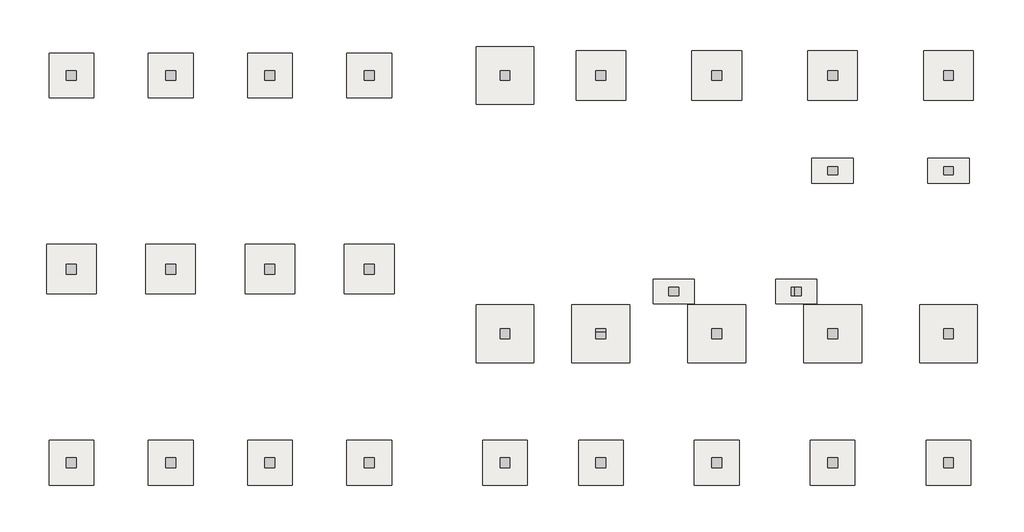
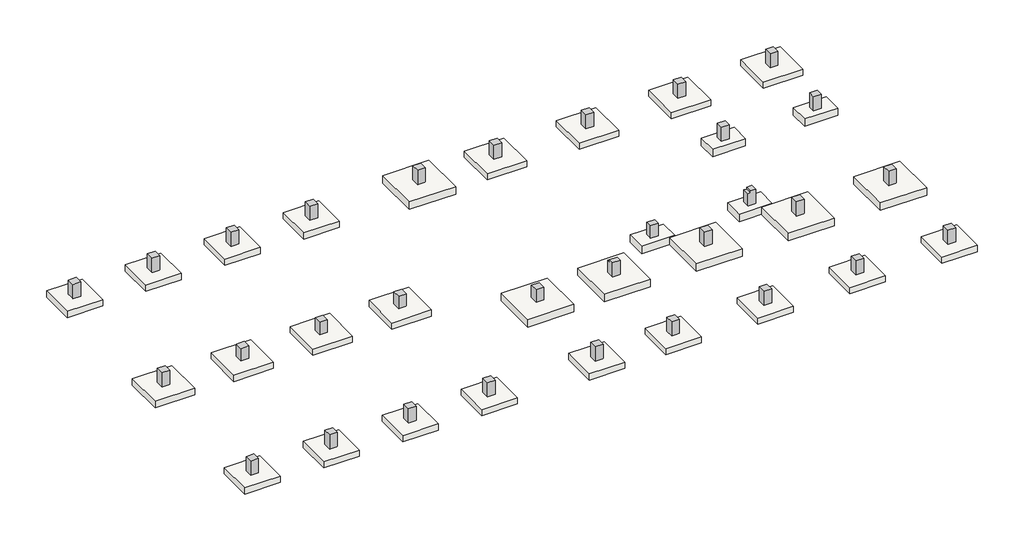
# Not in any storey: 31 columns, 31 slabs.
"""IFC4 building model written with IfcOpenShell, lengths in millimetres."""

import ifcopenshell
import ifcopenshell.guid

model = None  # the IFC model being written
_history = None  # IfcOwnerHistory: only IFC2X3 demands one
_inside = {}  # id of a spatial element -> (the spatial element, [elements in it])
_under = {}  # id of a project, library or spatial element -> (it, [spatial elements below it])
_declared = {}  # id of a project -> (the project, [libraries it declares])
_typed = {}  # id of a type object -> (the type object, [elements of that type])
_made_of = {}  # id of a material, layer set ... -> (it, [elements and type objects made of it])


def new_model(schema):
    """Start an empty IFC model of exactly this schema.

    Asked for "IFC4X3", IfcOpenShell would pick the latest addendum, in which some entities
    have other attributes; the version numbers below select the first issue.
    IFC2X3 requires an IfcOwnerHistory on every rooted entity: one is made here for all.
    """
    global model, _history
    if schema == "IFC4X3":
        model = ifcopenshell.file(schema_version=(4, 3, 0, 0))
    else:
        model = ifcopenshell.file(schema=schema)
    _inside.clear()
    _under.clear()
    _declared.clear()
    _typed.clear()
    _made_of.clear()
    _history = None
    if model.schema == "IFC2X3":
        org = make("IfcOrganization", Name="unknown")
        user = make(
            "IfcPersonAndOrganization",
            ThePerson=make("IfcPerson", FamilyName="unknown"),
            TheOrganization=org,
        )
        app = make(
            "IfcApplication",
            ApplicationDeveloper=org,
            Version="unknown",
            ApplicationFullName="unknown",
            ApplicationIdentifier="unknown",
        )
        _history = make(
            "IfcOwnerHistory",
            OwningUser=user,
            OwningApplication=app,
            ChangeAction="ADDED",
            CreationDate=0,
        )
    return model


def make(cls, **values):
    """One entity of the class cls with the attributes given. An attribute that is None is left unset."""
    return model.create_entity(
        cls, **{name: value for name, value in values.items() if value is not None}
    )


def rooted(cls, **values):
    """An entity with a GlobalId (a new one), such as an element, a storey or a relation."""
    return make(cls, GlobalId=ifcopenshell.guid.new(), OwnerHistory=_history, **values)


def si_unit(unit_type, name, prefix=None):
    """IfcSIUnit, for example si_unit("LENGTHUNIT", "METRE", prefix="MILLI")."""
    return make("IfcSIUnit", UnitType=unit_type, Prefix=prefix, Name=name)


def assignment(units):
    """IfcUnitAssignment: the units of a project."""
    return None if units is None else make("IfcUnitAssignment", Units=units)


def point(xyz):
    """IfcCartesianPoint."""
    return None if xyz is None else make("IfcCartesianPoint", Coordinates=xyz)


def direction(xyz):
    """IfcDirection."""
    return None if xyz is None else make("IfcDirection", DirectionRatios=xyz)


def frame(location, z_axis=None, x_axis=None):
    """IfcAxis2Placement3D, a coordinate frame: its origin and axes. An axis left out is left unset."""
    return make(
        "IfcAxis2Placement3D",
        Location=point(location),
        Axis=direction(z_axis),
        RefDirection=direction(x_axis),
    )


def origin():
    """The frame at (0, 0, 0) with its axes left unset."""
    return frame((0.0, 0.0, 0.0))


def place(relative_to, where):
    """IfcLocalPlacement: puts the frame where relative to a parent placement (None: the world)."""
    return make(
        "IfcLocalPlacement", PlacementRelTo=relative_to, RelativePlacement=where
    )


def context(
    kind, dimensions, precision=None, world=None, true_north=None, identifier=None
):
    """IfcGeometricRepresentationContext, for example the 3D "Model" context."""
    return make(
        "IfcGeometricRepresentationContext",
        ContextIdentifier=identifier,
        ContextType=kind,
        CoordinateSpaceDimension=dimensions,
        Precision=precision,
        WorldCoordinateSystem=world,
        TrueNorth=true_north,
    )


def project(units=None, contexts=None):
    """IfcProject with its units and contexts."""
    return rooted(
        "IfcProject",
        Name="project",
        RepresentationContexts=contexts,
        UnitsInContext=assignment(units),
    )


def spatial(cls, under=None, at=None, **own):
    """A site, building, storey or space (cls), placed at a placement, below another one or the project."""
    s = rooted(cls, ObjectPlacement=at, **own)
    if under is not None:
        _under.setdefault(under.id(), (under, []))[1].append(s)
    return s


def polyline(points):
    """IfcPolyline through the points."""
    return make("IfcPolyline", Points=[point(p) for p in points])


def outline(outer, holes=None, kind="AREA"):
    """IfcArbitraryClosedProfileDef: a profile drawn as a closed curve; with holes, ...WithVoids."""
    if holes is None:
        return make("IfcArbitraryClosedProfileDef", ProfileType=kind, OuterCurve=outer)
    return make(
        "IfcArbitraryProfileDefWithVoids",
        ProfileType=kind,
        OuterCurve=outer,
        InnerCurves=holes,
    )


def extrude(swept, where, along, depth):
    """IfcExtrudedAreaSolid: the profile swept, set in the frame where, extruded along a direction by depth."""
    return make(
        "IfcExtrudedAreaSolid",
        SweptArea=swept,
        Position=where,
        ExtrudedDirection=direction(along),
        Depth=depth,
    )


def faces_of(points, faces, orient=None, outer=None):
    """IfcFace entities. A face is a list of loops; a loop is a list of indices into points, from 0.

    orient and outer hold one flag for each loop. By default every Orientation is true, the
    first loop of a face is its IfcFaceOuterBound and the others are IfcFaceBound.
    """
    made = []
    for i, loops in enumerate(faces):
        bounds = []
        for j, loop in enumerate(loops):
            is_outer = j == 0 if outer is None else outer[i][j]
            bounds.append(
                make(
                    "IfcFaceOuterBound" if is_outer else "IfcFaceBound",
                    Bound=make("IfcPolyLoop", Polygon=[points[k] for k in loop]),
                    Orientation=True if orient is None else orient[i][j],
                )
            )
        made.append(make("IfcFace", Bounds=bounds))
    return made


def faceted_brep(points, faces, orient=None, outer=None, voids=None):
    """IfcFacetedBrep: a solid bounded by flat faces; with voids (closed shells), ...WithVoids."""
    shared = [point(p) for p in points]
    hull = make("IfcClosedShell", CfsFaces=faces_of(shared, faces, orient, outer))
    if voids is None:
        return make("IfcFacetedBrep", Outer=hull)
    return make(
        "IfcFacetedBrepWithVoids",
        Outer=hull,
        Voids=[
            make(cls, CfsFaces=faces_of(shared, fs, o, b)) for cls, fs, o, b in voids
        ],
    )


def shape(context_of_items, identifier, shape_type, items):
    """IfcShapeRepresentation: the items that make up one representation, for example the "Body"."""
    return make(
        "IfcShapeRepresentation",
        ContextOfItems=context_of_items,
        RepresentationIdentifier=identifier,
        RepresentationType=shape_type,
        Items=items,
    )


def made_of(thing, what):
    """Note that an element or type object is made of a material, layer set ...; save() writes the relation."""
    if what is not None:
        _made_of.setdefault(what.id(), (what, []))[1].append(thing)
    return thing


def element(
    cls,
    number,
    at=None,
    inside=None,
    cuts=None,
    type_object=None,
    material=None,
    context=None,
    identifier="Body",
    shape_type=None,
    held_by="IfcProductDefinitionShape",
    body=None,
    shapes=None,
    **own,
):
    """One element of the class cls, such as IfcWall. Its Tag is "e" and its number.

    at: its placement. inside: the storey or other place that contains it. cuts: it is an
    opening in that element (IfcRelVoidsElement). A single representation is given by context,
    identifier, shape_type and body (its items); several are given by shapes. held_by: the class
    of the entity that holds the representations. save() writes the other relations.
    """
    e = rooted(cls, Tag="e%d" % number, ObjectPlacement=at, **own)
    if body is not None:
        shapes = [shape(context, identifier, shape_type, body)]
    if shapes is not None:
        e.Representation = make(held_by, Representations=shapes)
    if inside is not None:
        _inside.setdefault(inside.id(), (inside, []))[1].append(e)
    if cuts is not None:
        rooted(
            "IfcRelVoidsElement", RelatingBuildingElement=cuts, RelatedOpeningElement=e
        )
    if type_object is not None:
        _typed.setdefault(type_object.id(), (type_object, []))[1].append(e)
    return made_of(e, material)


def aggregate(whole, parts):
    """IfcRelAggregates: a whole, such as a stair, and the parts it consists of."""
    return rooted("IfcRelAggregates", RelatingObject=whole, RelatedObjects=parts)


def save(model, path):
    """Write the relations noted so far, then the file.

    IfcRelAggregates (storeys below a building ...), IfcRelContainedInSpatialStructure (elements
    in a storey), IfcRelDefinesByType, IfcRelAssociatesMaterial and IfcRelDeclares: one each for
    every whole, place, type object, material and project.
    """
    for whole, parts in _under.values():
        aggregate(whole, parts)
    for where, things in _inside.values():
        rooted(
            "IfcRelContainedInSpatialStructure",
            RelatedElements=things,
            RelatingStructure=where,
        )
    for kind, things in _typed.values():
        rooted("IfcRelDefinesByType", RelatedObjects=things, RelatingType=kind)
    for what, things in _made_of.values():
        rooted("IfcRelAssociatesMaterial", RelatedObjects=things, RelatingMaterial=what)
    for by, libraries in _declared.values():
        rooted("IfcRelDeclares", RelatingContext=by, RelatedDefinitions=libraries)
    model.write(path)


model = new_model("IFC4")

# Units and contexts
model_context = context("Model", 3, world=origin())
ifc_project = project(units=[si_unit("LENGTHUNIT", "METRE", prefix="MILLI")], contexts=[model_context])

# Site, building
site = spatial("IfcSite", under=ifc_project)
building = spatial("IfcBuilding", under=site)

# Columns
placement = place(None, origin())
element("IfcColumn", 1, ObjectType="RC_Column_Rectangular : H_SC_AR_S15_UG PED_W600xL600_Bit", at=placement, inside=building, context=model_context, shape_type="Brep", body=[
    faceted_brep([(300.0, 12499.5208589, -1150.0381366), (300.0, 11899.5208589, -1150.0381366), (-300.0, 11899.5208589, -1150.0381366), (-300.0, 12499.5208589, -1150.0381366), (300.0, 12499.5208589, -0.0381366), (300.0, 11899.5208589, -0.0381366), (300.0, 11899.5208589, -150.0381366), (300.0, 11899.5208589, -650.0381366), (300.0, 12499.5208589, -650.0381366), (300.0, 12499.5208589, -150.0381366), (-300.0, 11899.5208589, -0.0381366), (-300.0, 11899.5208589, -150.0381366), (-300.0, 11899.5208589, -650.0381366), (-300.0, 12499.5208589, -0.0381366), (-300.0, 12499.5208589, -150.0381366), (-300.0, 12499.5208589, -650.0381366)], [[[0, 1, 2, 3]], [[4, 5, 6, 7, 1, 0, 8, 9]], [[5, 10, 11, 12, 2, 1, 7, 6]], [[10, 13, 14, 15, 3, 2, 12, 11]], [[13, 4, 9, 8, 0, 3, 15, 14]], [[4, 13, 10, 5]]]),
])
element("IfcColumn", 2, ObjectType="RC_Column_Rectangular : H_SC_AR_S15_UG PED_W600xL600_Bit", at=placement, inside=building, context=model_context, shape_type="SweptSolid", body=[
    extrude(outline(polyline([(6300.0, 12499.5208589), (6300.0, 11899.5208589), (5700.0, 11899.5208589), (5700.0, 12499.5208589), (6300.0, 12499.5208589)])), frame((0.0, 0.0, -1150.0381366), z_axis=(0.0, 0.0, 1.0), x_axis=(1.0, 0.0, 0.0)), (0.0, 0.0, 1.0), 1000.0),
])
element("IfcColumn", 3, ObjectType="RC_Column_Rectangular : H_SC_AR_S15_UG PED_W600xL600_Bit", at=placement, inside=building, context=model_context, shape_type="SweptSolid", body=[
    extrude(outline(polyline([(12300.0, 12499.5208589), (12300.0, 11899.5208589), (11700.0, 11899.5208589), (11700.0, 12499.5208589), (12300.0, 12499.5208589)])), frame((0.0, 0.0, -1150.0381366), z_axis=(0.0, 0.0, 1.0), x_axis=(1.0, 0.0, 0.0)), (0.0, 0.0, 1.0), 1000.0),
])
element("IfcColumn", 4, ObjectType="RC_Column_Rectangular : H_SC_AR_S15_UG PED_W600xL600_Bit", at=placement, inside=building, context=model_context, shape_type="Brep", body=[
    faceted_brep([(18300.0, 12499.5208589, -1150.0381366), (18300.0, 11899.5208589, -1150.0381366), (17700.0, 11899.5208589, -1150.0381366), (17700.0, 12499.5208589, -1150.0381366), (18300.0, 12499.5208589, -150.0381366), (18300.0, 11899.5208589, -150.0381366), (18200.0, 11899.5208589, -150.0381366), (17700.0, 11899.5208589, -150.0381366), (17700.0, 12499.5208589, -150.0381366)], [[[0, 1, 2, 3]], [[1, 0, 4, 5]], [[2, 1, 5, 6, 7]], [[3, 2, 7, 8]], [[0, 3, 8, 4]], [[5, 4, 8, 7, 6]]]),
])
element("IfcColumn", 5, ObjectType="RC_Column_Rectangular : H_SC_AR_S15_UG PED_W600xL600_Bit", at=placement, inside=building, context=model_context, shape_type="Brep", body=[
    faceted_brep([(300.0, 24199.5208589, -1150.0381366), (300.0, 23599.5208589, -1150.0381366), (-300.0, 23599.5208589, -1150.0381366), (-300.0, 24199.5208589, -1150.0381366), (300.0, 24199.5208589, -0.0381366), (300.0, 23599.5208589, -0.0381366), (300.0, 23599.5208589, -150.0381366), (300.0, 23599.5208589, -650.0381366), (300.0, 24199.5208589, -650.0381366), (300.0, 24199.5208589, -150.0381366), (-300.0, 23599.5208589, -0.0381366), (-300.0, 23599.5208589, -150.0381366), (-300.0, 23599.5208589, -650.0381366), (-300.0, 24199.5208589, -0.0381366)], [[[0, 1, 2, 3]], [[4, 5, 6, 7, 1, 0, 8, 9]], [[5, 10, 11, 12, 2, 1, 7, 6]], [[10, 13, 3, 2, 12, 11]], [[13, 4, 9, 8, 0, 3]], [[4, 13, 10, 5]]]),
])
element("IfcColumn", 6, ObjectType="RC_Column_Rectangular : H_SC_AR_S15_UG PED_W600xL600_Bit", at=placement, inside=building, context=model_context, shape_type="Brep", body=[
    faceted_brep([(6300.0, 24199.5208589, -1150.0381366), (6300.0, 23599.5208589, -1150.0381366), (5700.0, 23599.5208589, -1150.0381366), (5700.0, 24199.5208589, -1150.0381366), (6300.0, 24199.5208589, -0.0381366), (6300.0, 23599.5208589, -0.0381366), (6300.0, 23599.5208589, -150.0381366), (6300.0, 23599.5208589, -650.0381366), (6300.0, 24199.5208589, -650.0381366), (6300.0, 24199.5208589, -150.0381366), (5700.0, 23599.5208589, -0.0381366), (5700.0, 23599.5208589, -150.0381366), (5700.0, 23599.5208589, -650.0381366), (5700.0, 24199.5208589, -0.0381366), (5700.0, 24199.5208589, -150.0381366), (5700.0, 24199.5208589, -650.0381366)], [[[0, 1, 2, 3]], [[4, 5, 6, 7, 1, 0, 8, 9]], [[5, 10, 11, 12, 2, 1, 7, 6]], [[10, 13, 14, 15, 3, 2, 12, 11]], [[13, 4, 9, 8, 0, 3, 15, 14]], [[4, 13, 10, 5]]]),
])
element("IfcColumn", 7, ObjectType="RC_Column_Rectangular : H_SC_AR_S15_UG PED_W600xL600_Bit", at=placement, inside=building, context=model_context, shape_type="Brep", body=[
    faceted_brep([(12300.0, 24199.5208589, -1150.0381366), (12300.0, 23599.5208589, -1150.0381366), (11700.0, 23599.5208589, -1150.0381366), (11700.0, 24199.5208589, -1150.0381366), (12300.0, 24199.5208589, -0.0381366), (12300.0, 23599.5208589, -0.0381366), (12300.0, 23599.5208589, -150.0381366), (12300.0, 23599.5208589, -650.0381366), (12300.0, 24199.5208589, -650.0381366), (12300.0, 24199.5208589, -150.0381366), (11700.0, 23599.5208589, -0.0381366), (11700.0, 23599.5208589, -150.0381366), (11700.0, 23599.5208589, -650.0381366), (11700.0, 24199.5208589, -0.0381366), (11700.0, 24199.5208589, -150.0381366), (11700.0, 24199.5208589, -650.0381366)], [[[0, 1, 2, 3]], [[4, 5, 6, 7, 1, 0, 8, 9]], [[5, 10, 11, 12, 2, 1, 7, 6]], [[10, 13, 14, 15, 3, 2, 12, 11]], [[13, 4, 9, 8, 0, 3, 15, 14]], [[4, 13, 10, 5]]]),
])
element("IfcColumn", 8, ObjectType="RC_Column_Rectangular : H_SC_AR_S15_UG PED_W600xL600_Bit", at=placement, inside=building, context=model_context, shape_type="Brep", body=[
    faceted_brep([(18300.0, 24199.5208589, -1150.0381366), (18300.0, 23599.5208589, -1150.0381366), (17700.0, 23599.5208589, -1150.0381366), (17700.0, 24199.5208589, -1150.0381366), (18300.0, 24199.5208589, -0.0381366), (18300.0, 23599.5208589, -0.0381366), (18300.0, 23599.5208589, -150.0381366), (18300.0, 23599.5208589, -650.0381366), (18300.0, 24199.5208589, -650.0381366), (18300.0, 24199.5208589, -150.0381366), (17700.0, 23599.5208589, -0.0381366), (17700.0, 23599.5208589, -150.0381366), (17700.0, 23599.5208589, -650.0381366), (17700.0, 24199.5208589, -0.0381366), (17700.0, 24199.5208589, -150.0381366), (17700.0, 24199.5208589, -650.0381366)], [[[0, 1, 2, 3]], [[4, 5, 6, 7, 1, 0, 8, 9]], [[5, 10, 11, 12, 2, 1, 7, 6]], [[10, 13, 14, 15, 3, 2, 12, 11]], [[13, 4, 9, 8, 0, 3, 15, 14]], [[4, 13, 10, 5]]]),
])
element("IfcColumn", 9, ObjectType="RC_Column_Rectangular : H_SC_AR_S15_UG PED_W600xL600_Bit", at=placement, inside=building, context=model_context, shape_type="Brep", body=[
    faceted_brep([(26500.0, 24199.5208589, -1150.0381366), (26500.0, 23599.5208589, -1150.0381366), (25900.0, 23599.5208589, -1150.0381366), (25900.0, 24199.5208589, -1150.0381366), (26500.0, 24199.5208589, -0.0381366), (26500.0, 23599.5208589, -0.0381366), (26500.0, 23599.5208589, -150.0381366), (26500.0, 23599.5208589, -650.0381366), (26500.0, 24199.5208589, -650.0381366), (26500.0, 24199.5208589, -150.0381366), (25900.0, 23599.5208589, -0.0381366), (25900.0, 23599.5208589, -150.0381366), (25900.0, 23599.5208589, -650.0381366), (25900.0, 24199.5208589, -0.0381366), (25900.0, 24199.5208589, -150.0381366), (25900.0, 24199.5208589, -650.0381366)], [[[0, 1, 2, 3]], [[4, 5, 6, 7, 1, 0, 8, 9]], [[5, 10, 11, 12, 2, 1, 7, 6]], [[10, 13, 14, 15, 3, 2, 12, 11]], [[13, 4, 9, 8, 0, 3, 15, 14]], [[4, 13, 10, 5]]]),
])
element("IfcColumn", 10, ObjectType="RC_Column_Rectangular : H_SC_AR_S15_UG PED_W600xL600_Bit", at=placement, inside=building, context=model_context, shape_type="Brep", body=[
    faceted_brep([(32300.0, 24199.5208589, -1150.0381366), (32300.0, 23599.5208589, -1150.0381366), (31700.0, 23599.5208589, -1150.0381366), (31700.0, 24199.5208589, -1150.0381366), (32300.0, 24199.5208589, -0.0381366), (32300.0, 23599.5208589, -0.0381366), (32300.0, 23599.5208589, -150.0381366), (32300.0, 23599.5208589, -650.0381366), (32300.0, 24199.5208589, -650.0381366), (32300.0, 24199.5208589, -150.0381366), (31700.0, 23599.5208589, -0.0381366), (31700.0, 23599.5208589, -150.0381366), (31700.0, 23599.5208589, -650.0381366), (31700.0, 24199.5208589, -0.0381366), (31700.0, 24199.5208589, -150.0381366), (31700.0, 24199.5208589, -650.0381366)], [[[0, 1, 2, 3]], [[4, 5, 6, 7, 1, 0, 8, 9]], [[5, 10, 11, 12, 2, 1, 7, 6]], [[10, 13, 14, 15, 3, 2, 12, 11]], [[13, 4, 9, 8, 0, 3, 15, 14]], [[4, 13, 10, 5]]]),
])
element("IfcColumn", 11, ObjectType="RC_Column_Rectangular : H_SC_AR_S15_UG PED_W600xL600_Bit", at=placement, inside=building, context=model_context, shape_type="Brep", body=[
    faceted_brep([(39300.0, 24199.5208589, -1150.0381366), (39300.0, 23599.5208589, -1150.0381366), (38700.0, 23599.5208589, -1150.0381366), (38700.0, 24199.5208589, -1150.0381366), (39300.0, 24199.5208589, -0.0381366), (39300.0, 23599.5208589, -0.0381366), (39300.0, 23599.5208589, -150.0381366), (39300.0, 23599.5208589, -650.0381366), (39300.0, 24199.5208589, -650.0381366), (39300.0, 24199.5208589, -150.0381366), (38700.0, 23599.5208589, -0.0381366), (38700.0, 23599.5208589, -150.0381366), (38700.0, 23599.5208589, -650.0381366), (38700.0, 24199.5208589, -0.0381366), (38700.0, 24199.5208589, -150.0381366), (38700.0, 24199.5208589, -650.0381366)], [[[0, 1, 2, 3]], [[4, 5, 6, 7, 1, 0, 8, 9]], [[5, 10, 11, 12, 2, 1, 7, 6]], [[10, 13, 14, 15, 3, 2, 12, 11]], [[13, 4, 9, 8, 0, 3, 15, 14]], [[4, 13, 10, 5]]]),
])
element("IfcColumn", 12, ObjectType="RC_Column_Rectangular : H_SC_AR_S15_UG PED_W600xL600_Bit", at=placement, inside=building, context=model_context, shape_type="Brep", body=[
    faceted_brep([(46300.0, 24199.5208589, -1150.0381366), (46300.0, 23599.5208589, -1150.0381366), (45700.0, 23599.5208589, -1150.0381366), (45700.0, 24199.5208589, -1150.0381366), (46300.0, 24199.5208589, -0.0381366), (46300.0, 23599.5208589, -0.0381366), (46300.0, 23599.5208589, -150.0381366), (46300.0, 23599.5208589, -650.0381366), (46300.0, 24199.5208589, -650.0381366), (46300.0, 24199.5208589, -150.0381366), (45700.0, 23599.5208589, -0.0381366), (45700.0, 23599.5208589, -150.0381366), (45700.0, 23599.5208589, -650.0381366), (45700.0, 24199.5208589, -0.0381366), (45700.0, 24199.5208589, -150.0381366), (45700.0, 24199.5208589, -650.0381366)], [[[0, 1, 2, 3]], [[4, 5, 6, 7, 1, 0, 8, 9]], [[5, 10, 11, 12, 2, 1, 7, 6]], [[10, 13, 14, 15, 3, 2, 12, 11]], [[13, 4, 9, 8, 0, 3, 15, 14]], [[4, 13, 10, 5]]]),
])
element("IfcColumn", 13, ObjectType="RC_Column_Rectangular : H_SC_AR_S15_UG PED_W600xL600_Bit", at=placement, inside=building, context=model_context, shape_type="Brep", body=[
    faceted_brep([(53300.0, 24199.5208589, -1150.0381366), (53300.0, 23599.5208589, -1150.0381366), (52700.0, 23599.5208589, -1150.0381366), (52700.0, 24199.5208589, -1150.0381366), (53300.0, 24199.5208589, -0.0381366), (53300.0, 23599.5208589, -0.0381366), (53300.0, 23599.5208589, -150.0381366), (53300.0, 23599.5208589, -650.0381366), (52700.0, 23599.5208589, -0.0381366), (52700.0, 23599.5208589, -150.0381366), (52700.0, 23599.5208589, -650.0381366), (52700.0, 24199.5208589, -0.0381366), (52700.0, 24199.5208589, -150.0381366), (52700.0, 24199.5208589, -650.0381366)], [[[0, 1, 2, 3]], [[4, 5, 6, 7, 1, 0]], [[5, 8, 9, 10, 2, 1, 7, 6]], [[8, 11, 12, 13, 3, 2, 10, 9]], [[11, 4, 0, 3, 13, 12]], [[4, 11, 8, 5]]]),
])
element("IfcColumn", 14, ObjectType="RC_Column_Rectangular : H_SC_AR_S15_UG PED_W600xL600_Bit", at=placement, inside=building, context=model_context, shape_type="Brep", body=[
    faceted_brep([(26500.0, 8599.5208589, -1150.0381366), (26500.0, 7999.5208589, -1150.0381366), (25900.0, 7999.5208589, -1150.0381366), (25900.0, 8599.5208589, -1150.0381366), (26500.0, 8599.5208589, -150.0381366), (26500.0, 8399.5208589, -150.0381366), (26500.0, 7999.5208589, -150.0381366), (25900.0, 7999.5208589, -150.0381366), (25900.0, 8599.5208589, -150.0381366)], [[[0, 1, 2, 3]], [[1, 0, 4, 5, 6]], [[2, 1, 6, 7]], [[3, 2, 7, 8]], [[0, 3, 8, 4]], [[4, 8, 7, 6, 5]]]),
])
element("IfcColumn", 15, ObjectType="RC_Column_Rectangular : H_SC_AR_S15_UG PED_W600xL600_Bit", at=placement, inside=building, context=model_context, shape_type="Brep", body=[
    faceted_brep([(32300.0, 8599.5208589, -1150.0381366), (32300.0, 7999.5208589, -1150.0381366), (31700.0, 7999.5208589, -1150.0381366), (31700.0, 8599.5208589, -1150.0381366), (32300.0, 8599.5208589, -150.0381366), (32300.0, 8399.5208589, -150.0381366), (32300.0, 8399.5208589, -0.0381366), (32300.0, 7999.5208589, -0.0381366), (31700.0, 7999.5208589, -0.0381366), (31700.0, 8399.5208589, -0.0381366), (31700.0, 8399.5208589, -150.0381366), (31700.0, 8599.5208589, -150.0381366), (31800.0, 8399.5208589, -0.0381366), (31800.0, 8399.5208589, -150.0381366)], [[[0, 1, 2, 3]], [[1, 0, 4, 5, 6, 7]], [[2, 1, 7, 8]], [[3, 2, 8, 9, 10, 11]], [[0, 3, 11, 4]], [[8, 7, 6, 12, 9]], [[10, 13, 5, 4, 11]], [[5, 13, 12, 6]], [[13, 10, 9, 12]]]),
])
element("IfcColumn", 16, ObjectType="RC_Column_Rectangular : H_SC_AR_S15_UG PED_W600xL600_Bit", at=placement, inside=building, context=model_context, shape_type="SweptSolid", body=[
    extrude(outline(polyline([(39300.0, 8599.5208589), (39300.0, 7999.5208589), (38700.0, 7999.5208589), (38700.0, 8599.5208589), (39300.0, 8599.5208589)])), frame((0.0, 0.0, -1150.0381366), z_axis=(0.0, 0.0, 1.0), x_axis=(1.0, 0.0, 0.0)), (0.0, 0.0, 1.0), 1150.0),
])
element("IfcColumn", 17, ObjectType="RC_Column_Rectangular : H_SC_AR_S15_UG PED_W600xL600_Bit", at=placement, inside=building, context=model_context, shape_type="SweptSolid", body=[
    extrude(outline(polyline([(46300.0, 8599.5208589), (46300.0, 7999.5208589), (45700.0, 7999.5208589), (45700.0, 8599.5208589), (46300.0, 8599.5208589)])), frame((0.0, 0.0, -1150.0381366), z_axis=(0.0, 0.0, 1.0), x_axis=(1.0, 0.0, 0.0)), (0.0, 0.0, 1.0), 1150.0),
])
element("IfcColumn", 18, ObjectType="RC_Column_Rectangular : H_SC_AR_S15_UG PED_W600xL600_Bit", at=placement, inside=building, context=model_context, shape_type="Brep", body=[
    faceted_brep([(53300.0, 8599.5208589, -1150.0381366), (53300.0, 7999.5208589, -1150.0381366), (52700.0, 7999.5208589, -1150.0381366), (52700.0, 8599.5208589, -1150.0381366), (53300.0, 8599.5208589, -0.0381366), (53300.0, 7999.5208589, -0.0381366), (53300.0, 7999.5208589, -150.0381366), (53300.0, 7999.5208589, -650.0381366), (53300.0, 8599.5208589, -650.0381366), (53300.0, 8599.5208589, -150.0381366), (52700.0, 7999.5208589, -0.0381366), (52700.0, 7999.5208589, -150.0381366), (52700.0, 7999.5208589, -650.0381366), (52700.0, 8599.5208589, -0.0381366), (52700.0, 8599.5208589, -150.0381366), (52700.0, 8599.5208589, -650.0381366)], [[[0, 1, 2, 3]], [[4, 5, 6, 7, 1, 0, 8, 9]], [[5, 10, 11, 12, 2, 1, 7, 6]], [[10, 13, 14, 15, 3, 2, 12, 11]], [[13, 4, 9, 8, 0, 3, 15, 14]], [[4, 13, 10, 5]]]),
])
element("IfcColumn", 19, ObjectType="RC_Column_Rectangular : H_SC_AR_S15_UG PED_W600xL600_Bit", at=placement, inside=building, context=model_context, shape_type="Brep", body=[
    faceted_brep([(300.0, 799.5208589, -1150.0381366), (300.0, 199.5208589, -1150.0381366), (-300.0, 199.5208589, -1150.0381366), (-300.0, 799.5208589, -1150.0381366), (300.0, 799.5208589, -0.0381366), (300.0, 199.5208589, -0.0381366), (300.0, 199.5208589, -150.0381366), (300.0, 199.5208589, -650.0381366), (300.0, 799.5208589, -650.0381366), (300.0, 799.5208589, -150.0381366), (-300.0, 199.5208589, -0.0381366), (-300.0, 799.5208589, -0.0381366), (-300.0, 799.5208589, -150.0381366), (-300.0, 799.5208589, -650.0381366)], [[[0, 1, 2, 3]], [[4, 5, 6, 7, 1, 0, 8, 9]], [[5, 10, 2, 1, 7, 6]], [[10, 11, 12, 13, 3, 2]], [[11, 4, 9, 8, 0, 3, 13, 12]], [[4, 11, 10, 5]]]),
])
element("IfcColumn", 20, ObjectType="RC_Column_Rectangular : H_SC_AR_S15_UG PED_W600xL600_Bit", at=placement, inside=building, context=model_context, shape_type="Brep", body=[
    faceted_brep([(6300.0, 799.5208589, -1150.0381366), (6300.0, 199.5208589, -1150.0381366), (5700.0, 199.5208589, -1150.0381366), (5700.0, 799.5208589, -1150.0381366), (6300.0, 799.5208589, -0.0381366), (6300.0, 199.5208589, -0.0381366), (6300.0, 199.5208589, -150.0381366), (6300.0, 199.5208589, -650.0381366), (6300.0, 799.5208589, -650.0381366), (6300.0, 799.5208589, -150.0381366), (5700.0, 199.5208589, -0.0381366), (5700.0, 199.5208589, -150.0381366), (5700.0, 199.5208589, -650.0381366), (5700.0, 799.5208589, -0.0381366), (5700.0, 799.5208589, -150.0381366), (5700.0, 799.5208589, -650.0381366)], [[[0, 1, 2, 3]], [[4, 5, 6, 7, 1, 0, 8, 9]], [[5, 10, 11, 12, 2, 1, 7, 6]], [[10, 13, 14, 15, 3, 2, 12, 11]], [[13, 4, 9, 8, 0, 3, 15, 14]], [[4, 13, 10, 5]]]),
])
element("IfcColumn", 21, ObjectType="RC_Column_Rectangular : H_SC_AR_S15_UG PED_W600xL600_Bit", at=placement, inside=building, context=model_context, shape_type="Brep", body=[
    faceted_brep([(12300.0, 799.5208589, -1150.0381366), (12300.0, 199.5208589, -1150.0381366), (11700.0, 199.5208589, -1150.0381366), (11700.0, 799.5208589, -1150.0381366), (12300.0, 799.5208589, -0.0381366), (12300.0, 199.5208589, -0.0381366), (12300.0, 199.5208589, -150.0381366), (12300.0, 199.5208589, -650.0381366), (12300.0, 799.5208589, -650.0381366), (12300.0, 799.5208589, -150.0381366), (11700.0, 199.5208589, -0.0381366), (11700.0, 199.5208589, -150.0381366), (11700.0, 199.5208589, -650.0381366), (11700.0, 799.5208589, -0.0381366), (11700.0, 799.5208589, -150.0381366), (11700.0, 799.5208589, -650.0381366)], [[[0, 1, 2, 3]], [[4, 5, 6, 7, 1, 0, 8, 9]], [[5, 10, 11, 12, 2, 1, 7, 6]], [[10, 13, 14, 15, 3, 2, 12, 11]], [[13, 4, 9, 8, 0, 3, 15, 14]], [[4, 13, 10, 5]]]),
])
element("IfcColumn", 22, ObjectType="RC_Column_Rectangular : H_SC_AR_S15_UG PED_W600xL600_Bit", at=placement, inside=building, context=model_context, shape_type="Brep", body=[
    faceted_brep([(18300.0, 799.5208589, -1150.0381366), (18300.0, 199.5208589, -1150.0381366), (17700.0, 199.5208589, -1150.0381366), (17700.0, 799.5208589, -1150.0381366), (18300.0, 799.5208589, -0.0381366), (18300.0, 199.5208589, -0.0381366), (18300.0, 199.5208589, -150.0381366), (18300.0, 199.5208589, -650.0381366), (18300.0, 799.5208589, -650.0381366), (18300.0, 799.5208589, -150.0381366), (17700.0, 199.5208589, -0.0381366), (17700.0, 199.5208589, -150.0381366), (17700.0, 199.5208589, -650.0381366), (17700.0, 799.5208589, -0.0381366), (17700.0, 799.5208589, -150.0381366), (17700.0, 799.5208589, -650.0381366)], [[[0, 1, 2, 3]], [[4, 5, 6, 7, 1, 0, 8, 9]], [[5, 10, 11, 12, 2, 1, 7, 6]], [[10, 13, 14, 15, 3, 2, 12, 11]], [[13, 4, 9, 8, 0, 3, 15, 14]], [[4, 13, 10, 5]]]),
])
element("IfcColumn", 23, ObjectType="RC_Column_Rectangular : H_SC_AR_S15_UG PED_W600xL600_Bit", at=placement, inside=building, context=model_context, shape_type="Brep", body=[
    faceted_brep([(26500.0, 799.5208589, -1150.0381366), (26500.0, 199.5208589, -1150.0381366), (25900.0, 199.5208589, -1150.0381366), (25900.0, 799.5208589, -1150.0381366), (26500.0, 799.5208589, -0.0381366), (26500.0, 199.5208589, -0.0381366), (26500.0, 199.5208589, -150.0381366), (26500.0, 199.5208589, -650.0381366), (26500.0, 799.5208589, -650.0381366), (26500.0, 799.5208589, -150.0381366), (25900.0, 199.5208589, -0.0381366), (25900.0, 199.5208589, -150.0381366), (25900.0, 199.5208589, -650.0381366), (25900.0, 799.5208589, -0.0381366), (25900.0, 799.5208589, -150.0381366), (25900.0, 799.5208589, -650.0381366)], [[[0, 1, 2, 3]], [[4, 5, 6, 7, 1, 0, 8, 9]], [[5, 10, 11, 12, 2, 1, 7, 6]], [[10, 13, 14, 15, 3, 2, 12, 11]], [[13, 4, 9, 8, 0, 3, 15, 14]], [[4, 13, 10, 5]]]),
])
element("IfcColumn", 24, ObjectType="RC_Column_Rectangular : H_SC_AR_S15_UG PED_W600xL600_Bit", at=placement, inside=building, context=model_context, shape_type="Brep", body=[
    faceted_brep([(32300.0, 799.5208589, -1150.0381366), (32300.0, 199.5208589, -1150.0381366), (31700.0, 199.5208589, -1150.0381366), (31700.0, 799.5208589, -1150.0381366), (32300.0, 799.5208589, -0.0381366), (32300.0, 199.5208589, -0.0381366), (32300.0, 199.5208589, -150.0381366), (32300.0, 199.5208589, -650.0381366), (32300.0, 799.5208589, -650.0381366), (32300.0, 799.5208589, -150.0381366), (31700.0, 199.5208589, -0.0381366), (31700.0, 199.5208589, -150.0381366), (31700.0, 199.5208589, -650.0381366), (31700.0, 799.5208589, -0.0381366), (31700.0, 799.5208589, -150.0381366), (31700.0, 799.5208589, -650.0381366)], [[[0, 1, 2, 3]], [[4, 5, 6, 7, 1, 0, 8, 9]], [[5, 10, 11, 12, 2, 1, 7, 6]], [[10, 13, 14, 15, 3, 2, 12, 11]], [[13, 4, 9, 8, 0, 3, 15, 14]], [[4, 13, 10, 5]]]),
])
element("IfcColumn", 25, ObjectType="RC_Column_Rectangular : H_SC_AR_S15_UG PED_W600xL600_Bit", at=placement, inside=building, context=model_context, shape_type="Brep", body=[
    faceted_brep([(39300.0, 799.5208589, -1150.0381366), (39300.0, 199.5208589, -1150.0381366), (38700.0, 199.5208589, -1150.0381366), (38700.0, 799.5208589, -1150.0381366), (39300.0, 799.5208589, -0.0381366), (39300.0, 199.5208589, -0.0381366), (39300.0, 199.5208589, -150.0381366), (39300.0, 199.5208589, -650.0381366), (39300.0, 799.5208589, -650.0381366), (39300.0, 799.5208589, -150.0381366), (38700.0, 199.5208589, -0.0381366), (38700.0, 199.5208589, -150.0381366), (38700.0, 199.5208589, -650.0381366), (38700.0, 799.5208589, -0.0381366), (38700.0, 799.5208589, -150.0381366), (38700.0, 799.5208589, -650.0381366)], [[[0, 1, 2, 3]], [[4, 5, 6, 7, 1, 0, 8, 9]], [[5, 10, 11, 12, 2, 1, 7, 6]], [[10, 13, 14, 15, 3, 2, 12, 11]], [[13, 4, 9, 8, 0, 3, 15, 14]], [[4, 13, 10, 5]]]),
])
element("IfcColumn", 26, ObjectType="RC_Column_Rectangular : H_SC_AR_S15_UG PED_W600xL600_Bit", at=placement, inside=building, context=model_context, shape_type="Brep", body=[
    faceted_brep([(46300.0, 799.5208589, -1150.0381366), (46300.0, 199.5208589, -1150.0381366), (45700.0, 199.5208589, -1150.0381366), (45700.0, 799.5208589, -1150.0381366), (46300.0, 799.5208589, -0.0381366), (46300.0, 199.5208589, -0.0381366), (46300.0, 199.5208589, -150.0381366), (46300.0, 199.5208589, -650.0381366), (46300.0, 799.5208589, -650.0381366), (46300.0, 799.5208589, -150.0381366), (45700.0, 199.5208589, -0.0381366), (45700.0, 199.5208589, -150.0381366), (45700.0, 199.5208589, -650.0381366), (45700.0, 799.5208589, -0.0381366), (45700.0, 799.5208589, -150.0381366), (45700.0, 799.5208589, -650.0381366)], [[[0, 1, 2, 3]], [[4, 5, 6, 7, 1, 0, 8, 9]], [[5, 10, 11, 12, 2, 1, 7, 6]], [[10, 13, 14, 15, 3, 2, 12, 11]], [[13, 4, 9, 8, 0, 3, 15, 14]], [[4, 13, 10, 5]]]),
])
element("IfcColumn", 27, ObjectType="RC_Column_Rectangular : H_SC_AR_S15_UG PED_W600xL600_Bit", at=placement, inside=building, context=model_context, shape_type="Brep", body=[
    faceted_brep([(53300.0, 799.5208589, -1150.0381366), (53300.0, 199.5208589, -1150.0381366), (52700.0, 199.5208589, -1150.0381366), (52700.0, 799.5208589, -1150.0381366), (53300.0, 799.5208589, -0.0381366), (53300.0, 199.5208589, -0.0381366), (53300.0, 799.5208589, -650.0381366), (53300.0, 799.5208589, -150.0381366), (52700.0, 199.5208589, -0.0381366), (52700.0, 199.5208589, -150.0381366), (52700.0, 199.5208589, -650.0381366), (52700.0, 799.5208589, -0.0381366), (52700.0, 799.5208589, -150.0381366), (52700.0, 799.5208589, -650.0381366)], [[[0, 1, 2, 3]], [[4, 5, 1, 0, 6, 7]], [[5, 8, 9, 10, 2, 1]], [[8, 11, 12, 13, 3, 2, 10, 9]], [[11, 4, 7, 6, 0, 3, 13, 12]], [[4, 11, 8, 5]]]),
])
element("IfcColumn", 28, ObjectType="RC_Column_Rectangular : H_SC_AR_S15_UG PED_W600xL500_Bit_PD1A", at=placement, inside=building, context=model_context, shape_type="Brep", body=[
    faceted_brep([(52700.0, 18399.5208589, -1150.0381366), (53300.0, 18399.5208589, -1150.0381366), (53300.0, 17899.5208589, -1150.0381366), (52700.0, 17899.5208589, -1150.0381366), (52700.0, 18399.5208589, -0.0381366), (53300.0, 18399.5208589, -0.0381366), (53300.0, 18399.5208589, -150.0381366), (53300.0, 18399.5208589, -650.0381366), (52700.0, 18399.5208589, -650.0381366), (52700.0, 18399.5208589, -150.0381366), (53300.0, 17899.5208589, -0.0381366), (53300.0, 17899.5208589, -150.0381366), (53300.0, 17899.5208589, -650.0381366), (52700.0, 17899.5208589, -0.0381366), (52700.0, 17899.5208589, -150.0381366), (52700.0, 17899.5208589, -650.0381366)], [[[0, 1, 2, 3]], [[4, 5, 6, 7, 1, 0, 8, 9]], [[5, 10, 11, 12, 2, 1, 7, 6]], [[10, 13, 14, 15, 3, 2, 12, 11]], [[13, 4, 9, 8, 0, 3, 15, 14]], [[4, 13, 10, 5]]]),
])
element("IfcColumn", 29, ObjectType="RC_Column_Rectangular : H_SC_AR_S15_UG PED_W600xL500_Bit_PD1A", at=placement, inside=building, context=model_context, shape_type="SweptSolid", body=[
    extrude(outline(polyline([(45700.0, 18399.5208589), (46300.0, 18399.5208589), (46300.0, 17899.5208589), (45700.0, 17899.5208589), (45700.0, 18399.5208589)])), frame((0.0, 0.0, -1150.0381366), z_axis=(0.0, 0.0, 1.0), x_axis=(1.0, 0.0, 0.0)), (0.0, 0.0, 1.0), 1150.0),
])
element("IfcColumn", 30, ObjectType="RC_Column_Rectangular : H_SC_AR_S15_UG PED_W600xL500_Bit_PD1A", at=placement, inside=building, context=model_context, shape_type="SweptSolid", body=[
    extrude(outline(polyline([(36100.0, 11099.5208589), (36700.0, 11099.5208589), (36700.0, 10599.5208589), (36100.0, 10599.5208589), (36100.0, 11099.5208589)])), frame((0.0, 0.0, -1150.0381366), z_axis=(0.0, 0.0, 1.0), x_axis=(1.0, 0.0, 0.0)), (0.0, 0.0, 1.0), 1000.0),
])
element("IfcColumn", 31, ObjectType="RC_Column_Rectangular : H_SC_AR_S15_UG PED_W600xL500_Bit_PD1A", at=placement, inside=building, context=model_context, shape_type="SweptSolid", body=[
    extrude(outline(polyline([(-1150.0381366, 43500.0), (-1150.0381366, 44100.0), (-0.0381366, 44100.0), (-0.0381366, 43700.0), (-150.0381366, 43700.0), (-150.0381366, 43500.0), (-1150.0381366, 43500.0)])), frame((0.0, 10599.5208589, 0.0), z_axis=(0.0, 1.0, 0.0), x_axis=(0.0, 0.0, 1.0)), (0.0, 0.0, 1.0), 500.0),
])

# Slabs
element("IfcSlab", 32, ObjectType="Foundation Rectangular (Non-Pile) : H_SF_AR_S18_W3000xL3000xT500_Bitumen_F2", at=placement, inside=building, context=model_context, shape_type="SweptSolid", body=[
    extrude(outline(polyline([(1500.0, 13699.5208589), (1500.0, 10699.5208589), (-1500.0, 10699.5208589), (-1500.0, 13699.5208589), (1500.0, 13699.5208589)])), frame((0.0, 0.0, -1650.0381366), z_axis=(0.0, 0.0, 1.0), x_axis=(1.0, 0.0, 0.0)), (0.0, 0.0, 1.0), 500.0),
])
element("IfcSlab", 33, ObjectType="Foundation Rectangular (Non-Pile) : H_SF_AR_S18_W3000xL3000xT500_Bitumen_F2", at=placement, inside=building, context=model_context, shape_type="SweptSolid", body=[
    extrude(outline(polyline([(7500.0, 13699.5208589), (7500.0, 10699.5208589), (4500.0, 10699.5208589), (4500.0, 13699.5208589), (7500.0, 13699.5208589)])), frame((0.0, 0.0, -1650.0381366), z_axis=(0.0, 0.0, 1.0), x_axis=(1.0, 0.0, 0.0)), (0.0, 0.0, 1.0), 500.0),
])
element("IfcSlab", 34, ObjectType="Foundation Rectangular (Non-Pile) : H_SF_AR_S18_W3000xL3000xT500_Bitumen_F2", at=placement, inside=building, context=model_context, shape_type="SweptSolid", body=[
    extrude(outline(polyline([(13500.0, 13699.5208589), (13500.0, 10699.5208589), (10500.0, 10699.5208589), (10500.0, 13699.5208589), (13500.0, 13699.5208589)])), frame((0.0, 0.0, -1650.0381366), z_axis=(0.0, 0.0, 1.0), x_axis=(1.0, 0.0, 0.0)), (0.0, 0.0, 1.0), 500.0),
])
element("IfcSlab", 35, ObjectType="Foundation Rectangular (Non-Pile) : H_SF_AR_S18_W3000xL3000xT500_Bitumen_F2", at=placement, inside=building, context=model_context, shape_type="SweptSolid", body=[
    extrude(outline(polyline([(19500.0, 13699.5208589), (19500.0, 10699.5208589), (16500.0, 10699.5208589), (16500.0, 13699.5208589), (19500.0, 13699.5208589)])), frame((0.0, 0.0, -1650.0381366), z_axis=(0.0, 0.0, 1.0), x_axis=(1.0, 0.0, 0.0)), (0.0, 0.0, 1.0), 500.0),
])
element("IfcSlab", 36, ObjectType="Foundation Rectangular (Non-Pile) : H_SF_AR_S18_W2700xL2700xT500_Bitumen_F1", at=placement, inside=building, context=model_context, shape_type="SweptSolid", body=[
    extrude(outline(polyline([(1350.0, 25249.5208589), (1350.0, 22549.5208589), (-1350.0, 22549.5208589), (-1350.0, 25249.5208589), (1350.0, 25249.5208589)])), frame((0.0, 0.0, -1650.0381366), z_axis=(0.0, 0.0, 1.0), x_axis=(1.0, 0.0, 0.0)), (0.0, 0.0, 1.0), 500.0),
])
element("IfcSlab", 37, ObjectType="Foundation Rectangular (Non-Pile) : H_SF_AR_S18_W2700xL2700xT500_Bitumen_F1", at=placement, inside=building, context=model_context, shape_type="SweptSolid", body=[
    extrude(outline(polyline([(7350.0, 25249.5208589), (7350.0, 22549.5208589), (4650.0, 22549.5208589), (4650.0, 25249.5208589), (7350.0, 25249.5208589)])), frame((0.0, 0.0, -1650.0381366), z_axis=(0.0, 0.0, 1.0), x_axis=(1.0, 0.0, 0.0)), (0.0, 0.0, 1.0), 500.0),
])
element("IfcSlab", 38, ObjectType="Foundation Rectangular (Non-Pile) : H_SF_AR_S18_W2700xL2700xT500_Bitumen_F1", at=placement, inside=building, context=model_context, shape_type="SweptSolid", body=[
    extrude(outline(polyline([(13350.0, 25249.5208589), (13350.0, 22549.5208589), (10650.0, 22549.5208589), (10650.0, 25249.5208589), (13350.0, 25249.5208589)])), frame((0.0, 0.0, -1650.0381366), z_axis=(0.0, 0.0, 1.0), x_axis=(1.0, 0.0, 0.0)), (0.0, 0.0, 1.0), 500.0),
])
element("IfcSlab", 39, ObjectType="Foundation Rectangular (Non-Pile) : H_SF_AR_S18_W2700xL2700xT500_Bitumen_F1", at=placement, inside=building, context=model_context, shape_type="SweptSolid", body=[
    extrude(outline(polyline([(19350.0, 25249.5208589), (19350.0, 22549.5208589), (16650.0, 22549.5208589), (16650.0, 25249.5208589), (19350.0, 25249.5208589)])), frame((0.0, 0.0, -1650.0381366), z_axis=(0.0, 0.0, 1.0), x_axis=(1.0, 0.0, 0.0)), (0.0, 0.0, 1.0), 500.0),
])
element("IfcSlab", 40, ObjectType="Foundation Rectangular (Non-Pile) : H_SF_AR_S18_W3500xL3500xT600_Bitumen_F3", at=placement, inside=building, context=model_context, shape_type="SweptSolid", body=[
    extrude(outline(polyline([(27950.0, 25649.5208589), (27950.0, 22149.5208589), (24450.0, 22149.5208589), (24450.0, 25649.5208589), (27950.0, 25649.5208589)])), frame((0.0, 0.0, -1750.0381366), z_axis=(0.0, 0.0, 1.0), x_axis=(1.0, 0.0, 0.0)), (0.0, 0.0, 1.0), 600.0),
])
element("IfcSlab", 41, ObjectType="Foundation Rectangular (Non-Pile) : H_SF_AR_S18_W3000xL3000xT500_Bitumen_F2A", at=placement, inside=building, context=model_context, shape_type="SweptSolid", body=[
    extrude(outline(polyline([(33500.0, 25399.5208589), (33500.0, 22399.5208589), (30500.0, 22399.5208589), (30500.0, 25399.5208589), (33500.0, 25399.5208589)])), frame((0.0, 0.0, -1650.0381366), z_axis=(0.0, 0.0, 1.0), x_axis=(1.0, 0.0, 0.0)), (0.0, 0.0, 1.0), 500.0),
])
element("IfcSlab", 42, ObjectType="Foundation Rectangular (Non-Pile) : H_SF_AR_S18_W3000xL3000xT500_Bitumen_F2A", at=placement, inside=building, context=model_context, shape_type="SweptSolid", body=[
    extrude(outline(polyline([(40500.0, 25399.5208589), (40500.0, 22399.5208589), (37500.0, 22399.5208589), (37500.0, 25399.5208589), (40500.0, 25399.5208589)])), frame((0.0, 0.0, -1650.0381366), z_axis=(0.0, 0.0, 1.0), x_axis=(1.0, 0.0, 0.0)), (0.0, 0.0, 1.0), 500.0),
])
element("IfcSlab", 43, ObjectType="Foundation Rectangular (Non-Pile) : H_SF_AR_S18_W3000xL3000xT500_Bitumen_F2A", at=placement, inside=building, context=model_context, shape_type="SweptSolid", body=[
    extrude(outline(polyline([(47500.0, 25399.5208589), (47500.0, 22399.5208589), (44500.0, 22399.5208589), (44500.0, 25399.5208589), (47500.0, 25399.5208589)])), frame((0.0, 0.0, -1650.0381366), z_axis=(0.0, 0.0, 1.0), x_axis=(1.0, 0.0, 0.0)), (0.0, 0.0, 1.0), 500.0),
])
element("IfcSlab", 44, ObjectType="Foundation Rectangular (Non-Pile) : H_SF_AR_S18_W3000xL3000xT500_Bitumen_F2A", at=placement, inside=building, context=model_context, shape_type="SweptSolid", body=[
    extrude(outline(polyline([(54500.0, 25399.5208589), (54500.0, 22399.5208589), (51500.0, 22399.5208589), (51500.0, 25399.5208589), (54500.0, 25399.5208589)])), frame((0.0, 0.0, -1650.0381366), z_axis=(0.0, 0.0, 1.0), x_axis=(1.0, 0.0, 0.0)), (0.0, 0.0, 1.0), 500.0),
])
element("IfcSlab", 45, ObjectType="Foundation Rectangular (Non-Pile) : H_SF_AR_S18_W3500xL3500xT600_Bitumen_F3", at=placement, inside=building, context=model_context, shape_type="SweptSolid", body=[
    extrude(outline(polyline([(27950.0, 10049.5208589), (27950.0, 6549.5208589), (24450.0, 6549.5208589), (24450.0, 10049.5208589), (27950.0, 10049.5208589)])), frame((0.0, 0.0, -1750.0381366), z_axis=(0.0, 0.0, 1.0), x_axis=(1.0, 0.0, 0.0)), (0.0, 0.0, 1.0), 600.0),
])
element("IfcSlab", 46, ObjectType="Foundation Rectangular (Non-Pile) : H_SF_AR_S18_W3500xL3500xT600_Bitumen_F3", at=placement, inside=building, context=model_context, shape_type="SweptSolid", body=[
    extrude(outline(polyline([(33750.0, 10049.5208589), (33750.0, 6549.5208589), (30250.0, 6549.5208589), (30250.0, 10049.5208589), (33750.0, 10049.5208589)])), frame((0.0, 0.0, -1750.0381366), z_axis=(0.0, 0.0, 1.0), x_axis=(1.0, 0.0, 0.0)), (0.0, 0.0, 1.0), 600.0),
])
element("IfcSlab", 47, ObjectType="Foundation Rectangular (Non-Pile) : H_SF_AR_S18_W3500xL3500xT600_Bitumen_F3", at=placement, inside=building, context=model_context, shape_type="SweptSolid", body=[
    extrude(outline(polyline([(40750.0, 10049.5208589), (40750.0, 6549.5208589), (37250.0, 6549.5208589), (37250.0, 10049.5208589), (40750.0, 10049.5208589)])), frame((0.0, 0.0, -1750.0381366), z_axis=(0.0, 0.0, 1.0), x_axis=(1.0, 0.0, 0.0)), (0.0, 0.0, 1.0), 600.0),
])
element("IfcSlab", 48, ObjectType="Foundation Rectangular (Non-Pile) : H_SF_AR_S18_W3500xL3500xT600_Bitumen_F3", at=placement, inside=building, context=model_context, shape_type="SweptSolid", body=[
    extrude(outline(polyline([(47750.0, 10049.5208589), (47750.0, 6549.5208589), (44250.0, 6549.5208589), (44250.0, 10049.5208589), (47750.0, 10049.5208589)])), frame((0.0, 0.0, -1750.0381366), z_axis=(0.0, 0.0, 1.0), x_axis=(1.0, 0.0, 0.0)), (0.0, 0.0, 1.0), 600.0),
])
element("IfcSlab", 49, ObjectType="Foundation Rectangular (Non-Pile) : H_SF_AR_S18_W3500xL3500xT600_Bitumen_F3", at=placement, inside=building, context=model_context, shape_type="SweptSolid", body=[
    extrude(outline(polyline([(54750.0, 10049.5208589), (54750.0, 6549.5208589), (51250.0, 6549.5208589), (51250.0, 10049.5208589), (54750.0, 10049.5208589)])), frame((0.0, 0.0, -1750.0381366), z_axis=(0.0, 0.0, 1.0), x_axis=(1.0, 0.0, 0.0)), (0.0, 0.0, 1.0), 600.0),
])
element("IfcSlab", 50, ObjectType="Foundation Rectangular (Non-Pile) : H_SF_AR_S18_W2700xL2700xT500_Bitumen_F1A", at=placement, inside=building, context=model_context, shape_type="SweptSolid", body=[
    extrude(outline(polyline([(1350.0, 1849.5208589), (1350.0, -850.4791411), (-1350.0, -850.4791411), (-1350.0, 1849.5208589), (1350.0, 1849.5208589)])), frame((0.0, 0.0, -1650.0381366), z_axis=(0.0, 0.0, 1.0), x_axis=(1.0, 0.0, 0.0)), (0.0, 0.0, 1.0), 500.0),
])
element("IfcSlab", 51, ObjectType="Foundation Rectangular (Non-Pile) : H_SF_AR_S18_W2700xL2700xT500_Bitumen_F1", at=placement, inside=building, context=model_context, shape_type="SweptSolid", body=[
    extrude(outline(polyline([(7350.0, 1849.5208589), (7350.0, -850.4791411), (4650.0, -850.4791411), (4650.0, 1849.5208589), (7350.0, 1849.5208589)])), frame((0.0, 0.0, -1650.0381366), z_axis=(0.0, 0.0, 1.0), x_axis=(1.0, 0.0, 0.0)), (0.0, 0.0, 1.0), 500.0),
])
element("IfcSlab", 52, ObjectType="Foundation Rectangular (Non-Pile) : H_SF_AR_S18_W2700xL2700xT500_Bitumen_F1", at=placement, inside=building, context=model_context, shape_type="SweptSolid", body=[
    extrude(outline(polyline([(13350.0, 1849.5208589), (13350.0, -850.4791411), (10650.0, -850.4791411), (10650.0, 1849.5208589), (13350.0, 1849.5208589)])), frame((0.0, 0.0, -1650.0381366), z_axis=(0.0, 0.0, 1.0), x_axis=(1.0, 0.0, 0.0)), (0.0, 0.0, 1.0), 500.0),
])
element("IfcSlab", 53, ObjectType="Foundation Rectangular (Non-Pile) : H_SF_AR_S18_W2700xL2700xT500_Bitumen_F1", at=placement, inside=building, context=model_context, shape_type="SweptSolid", body=[
    extrude(outline(polyline([(19350.0, 1849.5208589), (19350.0, -850.4791411), (16650.0, -850.4791411), (16650.0, 1849.5208589), (19350.0, 1849.5208589)])), frame((0.0, 0.0, -1650.0381366), z_axis=(0.0, 0.0, 1.0), x_axis=(1.0, 0.0, 0.0)), (0.0, 0.0, 1.0), 500.0),
])
element("IfcSlab", 54, ObjectType="Foundation Rectangular (Non-Pile) : H_SF_AR_S18_W2700xL2700xT500_Bitumen_F1A", at=placement, inside=building, context=model_context, shape_type="SweptSolid", body=[
    extrude(outline(polyline([(27550.0, 1849.5208589), (27550.0, -850.4791411), (24850.0, -850.4791411), (24850.0, 1849.5208589), (27550.0, 1849.5208589)])), frame((0.0, 0.0, -1650.0381366), z_axis=(0.0, 0.0, 1.0), x_axis=(1.0, 0.0, 0.0)), (0.0, 0.0, 1.0), 500.0),
])
element("IfcSlab", 55, ObjectType="Foundation Rectangular (Non-Pile) : H_SF_AR_S18_W2700xL2700xT500_Bitumen_F1A", at=placement, inside=building, context=model_context, shape_type="SweptSolid", body=[
    extrude(outline(polyline([(33350.0, 1849.5208589), (33350.0, -850.4791411), (30650.0, -850.4791411), (30650.0, 1849.5208589), (33350.0, 1849.5208589)])), frame((0.0, 0.0, -1650.0381366), z_axis=(0.0, 0.0, 1.0), x_axis=(1.0, 0.0, 0.0)), (0.0, 0.0, 1.0), 500.0),
])
element("IfcSlab", 56, ObjectType="Foundation Rectangular (Non-Pile) : H_SF_AR_S18_W2700xL2700xT500_Bitumen_F1", at=placement, inside=building, context=model_context, shape_type="SweptSolid", body=[
    extrude(outline(polyline([(40350.0, 1849.5208589), (40350.0, -850.4791411), (37650.0, -850.4791411), (37650.0, 1849.5208589), (40350.0, 1849.5208589)])), frame((0.0, 0.0, -1650.0381366), z_axis=(0.0, 0.0, 1.0), x_axis=(1.0, 0.0, 0.0)), (0.0, 0.0, 1.0), 500.0),
])
element("IfcSlab", 57, ObjectType="Foundation Rectangular (Non-Pile) : H_SF_AR_S18_W2700xL2700xT500_Bitumen_F1", at=placement, inside=building, context=model_context, shape_type="SweptSolid", body=[
    extrude(outline(polyline([(47350.0, 1849.5208589), (47350.0, -850.4791411), (44650.0, -850.4791411), (44650.0, 1849.5208589), (47350.0, 1849.5208589)])), frame((0.0, 0.0, -1650.0381366), z_axis=(0.0, 0.0, 1.0), x_axis=(1.0, 0.0, 0.0)), (0.0, 0.0, 1.0), 500.0),
])
element("IfcSlab", 58, ObjectType="Foundation Rectangular (Non-Pile) : H_SF_AR_S18_W2700xL2700xT500_Bitumen_F1", at=placement, inside=building, context=model_context, shape_type="SweptSolid", body=[
    extrude(outline(polyline([(54350.0, 1849.5208589), (54350.0, -850.4791411), (51650.0, -850.4791411), (51650.0, 1849.5208589), (54350.0, 1849.5208589)])), frame((0.0, 0.0, -1650.0381366), z_axis=(0.0, 0.0, 1.0), x_axis=(1.0, 0.0, 0.0)), (0.0, 0.0, 1.0), 500.0),
])
element("IfcSlab", 59, ObjectType="Foundation Rectangular (Non-Pile) : H_SF_AR_S18_W2500xL1500xT600_Bitumen_F4", at=placement, inside=building, context=model_context, shape_type="SweptSolid", body=[
    extrude(outline(polyline([(47250.0, 18899.5208589), (47250.0, 17399.5208589), (44750.0, 17399.5208589), (44750.0, 18899.5208589), (47250.0, 18899.5208589)])), frame((0.0, 0.0, -1750.0381366), z_axis=(0.0, 0.0, 1.0), x_axis=(1.0, 0.0, 0.0)), (0.0, 0.0, 1.0), 600.0),
])
element("IfcSlab", 60, ObjectType="Foundation Rectangular (Non-Pile) : H_SF_AR_S18_W2500xL1500xT600_Bitumen_F4", at=placement, inside=building, context=model_context, shape_type="SweptSolid", body=[
    extrude(outline(polyline([(54250.0, 18899.5208589), (54250.0, 17399.5208589), (51750.0, 17399.5208589), (51750.0, 18899.5208589), (54250.0, 18899.5208589)])), frame((0.0, 0.0, -1750.0381366), z_axis=(0.0, 0.0, 1.0), x_axis=(1.0, 0.0, 0.0)), (0.0, 0.0, 1.0), 600.0),
])
element("IfcSlab", 61, ObjectType="Foundation Rectangular (Non-Pile) : H_SF_AR_S18_W2500xL1500xT600_Bitumen_F4", at=placement, inside=building, context=model_context, shape_type="SweptSolid", body=[
    extrude(outline(polyline([(37650.0, 11599.5208589), (37650.0, 10099.5208589), (35150.0, 10099.5208589), (35150.0, 11599.5208589), (37650.0, 11599.5208589)])), frame((0.0, 0.0, -1750.0381366), z_axis=(0.0, 0.0, 1.0), x_axis=(1.0, 0.0, 0.0)), (0.0, 0.0, 1.0), 600.0),
])
element("IfcSlab", 62, ObjectType="Foundation Rectangular (Non-Pile) : H_SF_AR_S18_W2500xL1500xT600_Bitumen_F4", at=placement, inside=building, context=model_context, shape_type="SweptSolid", body=[
    extrude(outline(polyline([(45050.0, 11599.5208589), (45050.0, 10099.5208589), (42550.0, 10099.5208589), (42550.0, 11599.5208589), (45050.0, 11599.5208589)])), frame((0.0, 0.0, -1750.0381366), z_axis=(0.0, 0.0, 1.0), x_axis=(1.0, 0.0, 0.0)), (0.0, 0.0, 1.0), 600.0),
])

save(model, "model.ifc")

# Revit data of these elements
# Type "RC_Column_Rectangular : H_SC_AR_S15_UG PED_W600xL600_Bit"
#   H_Q'ty Cal Type Tag = "SC-Q1A"
#   H_WM Code_1 = "A03AD044-00001 |  | M | Concrete Work | Substructure Work | Isolation Joint (Separation Joint) | w/ Flexible Joint Filler, Sealant | THK=(  )mm | A03AD044-00001 Concrete Work Substructure Work Isolation Joint (Separation Joint)      w/ Flexible Joint Filler, Sealant   | THK=( 12 )mm"
#   H_WM Code_2 = "A03AD032-00012 |  | M3 | Concrete Work | Substructure Work | Structural Concrete | Cement Type-5 | 20MPa < F'c (Cylinder Strength) ≤ 25MPa |  |  |  | A03AD032-00012 Concrete Work Substructure Work Structural Concrete  Cement Type-5 20MPa < F'c (Cylinder Strength) ≤ 25MPa      |  F'c (Cylinder Strength) = 24MPa"
#   H_WM Code_3 = "A03AD037-00002 |  | TON | Concrete Work | Substructure Work | Rebar Work | Deformed Bar (Non-Coat.) | 400MPa<Fy≤470MPa |  |  |  | A03AD037-00002 Concrete Work Substructure Work Rebar Work Deformed Bar (Non-Coat.)  400MPa<Fy≤470MPa      | ASTM A615 GRADE 60 (Fy=420MPa)"
#   H_WM Code_4 = "A03AD035-00001 |  | M2 | Concrete Work | Substructure Work | Form Work (3 times in use) | Flat Form | Dressed Lumber, Plywood or Steel Form(Wood Planks are not Allowed) incl. Chamfer |  |  | A03AD035-00001 Concrete Work Substructure Work Form Work (3 times in use) Flat Form     Dressed Lumber, Plywood or Steel Form(Wood Planks are not Allowed) incl. Chamfer   |"
#   H_WM Code_5 = "A03AH056-00001 |  | M2 | Concrete Work | Concrete Protective Coating (U/G) | Bitumen/Bituminous/Asphalt Coating |  | A03AH056-00001 Concrete Work Concrete Protective Coating (U/G) Bitumen/Bituminous/Asphalt Coating         |"
#   Width = 600 mm
#   Length = 600 mm
#   hec_material3 [instance default] = none
#   hec_material2 [instance default] = none
#   hec_material1 [instance default] = none
#   Structural Material [instance default] = none
#   Description = (empty or 0)
# Type "RC_Column_Rectangular : H_SC_AR_S15_UG PED_W600xL500_Bit_PD1A"
#   H_Q'ty Cal Type Tag = "SC-Q1"
#   H_WM Code_1 = "A03AF032-00010 |  | M3 | Concrete Work | Superstructure Work | Structural Concrete | Cement Type-1 | 20MPa < F'c (Cylinder Strength) ≤ 25MPa |  |  |  | A03AF032-00010 Concrete Work Superstructure Work Structural Concrete  Cement Type-1 20MPa < F'c (Cylinder Strength) ≤ 25MPa      |  F'c (Cylinder Strength) = 24MPa"
#   H_WM Code_2 = "A03AD037-00002 |  | TON | Concrete Work | Substructure Work | Rebar Work | Deformed Bar (Non-Coat.) | 400MPa<Fy≤470MPa |  |  |  | A03AD037-00002 Concrete Work Substructure Work Rebar Work Deformed Bar (Non-Coat.)  400MPa<Fy≤470MPa      | ASTM A615 GRADE 60 (Fy=420MPa)"
#   H_WM Code_3 = "A03AF036-00001 |  | M2 | Concrete Work | Superstructure Work | Form Work (1 time in use) | Flat Form | Dressed Lumber, Plywood or Steel Form(Wood Planks are not Allowed) incl. Chamfer |  |  | A03AF036-00001 Concrete Work Superstructure Work Form Work (1 time in use) Flat Form     Dressed Lumber, Plywood or Steel Form(Wood Planks are not Allowed) incl. Chamfer   |"
#   H_WM Code_4 = "A04AM077-00001 |  | M2 | Finishing Work | Painting Work | External Wall Painting | Acrylic Emulsion Paint |  |  |  | A04AM077-00001 Finishing Work Painting Work External Wall Painting Acrylic Emulsion Paint        |"
#   Width = 500 mm
#   Length = 600 mm
#   hec_material3 [instance default] = none
#   hec_material2 [instance default] = none
#   hec_material1 [instance default] = none
#   Structural Material [instance default] = none
#   Description = (empty or 0)
# Type "Foundation Rectangular (Non-Pile) : H_SF_AR_S18_W3000xL3000xT500_Bitumen_F2"
#   H_Q'ty Cal Type Tag = "SF-Q4"
#   H_WM Code_1 = "A03AD032-00010 |  | M3 | Concrete Work | Substructure Work | Structural Concrete | Cement Type-1 | 20MPa < F'c (Cylinder Strength) ≤ 25MPa |  |  |  | A03AD032-00010 Concrete Work Substructure Work Structural Concrete  Cement Type-1 20MPa < F'c (Cylinder Strength) ≤ 25MPa      |  F'c (Cylinder Strength) = 24MPa"
#   H_WM Code_2 = "A03AD037-00002 |  | TON | Concrete Work | Substructure Work | Rebar Work | Deformed Bar (Non-Coat.) | 400MPa<Fy≤470MPa |  |  |  | A03AD037-00002 Concrete Work Substructure Work Rebar Work Deformed Bar (Non-Coat.)  400MPa<Fy≤470MPa      | ASTM A615 GRADE 60 (Fy=420MPa)"
#   H_WM Code_3 = "A03AD035-00001 |  | M2 | Concrete Work | Substructure Work | Form Work (3 times in use) | Flat Form | Dressed Lumber, Plywood or Steel Form(Wood Planks are not Allowed) incl. Chamfer |  |  | A03AD035-00001 Concrete Work Substructure Work Form Work (3 times in use) Flat Form     Dressed Lumber, Plywood or Steel Form(Wood Planks are not Allowed) incl. Chamfer   |"
#   H_WM Code_4 = "A03AH056-00001 |  | M2 | Concrete Work | Concrete Protective Coating (U/G) | Bitumen/Bituminous/Asphalt Coating |  | A03AH056-00001 Concrete Work Concrete Protective Coating (U/G) Bitumen/Bituminous/Asphalt Coating         |"
#   H_WM Code_5 = "A01ZZ001-00004 |  | M3 | Earth Work | - | Excavation | Soil, Mech. |  | D ≤ 2.0M |  |  | A01ZZ001-00004 Earth Work - Excavation Soil, Mech.      D ≤ 2.0M  | D=2.0m"
#   H_WM Code_6 = "A01ZZ003-00001 |  | M3 | Earth Work | - | Backfill | Re-use, Soil |  |  |  | Compaction=(  )% | A01ZZ003-00001 Earth Work - Backfill Re-use, Soil        | Compaction=( 95 )%"
#   H_WM Code_7 = "A01ZZ004-00001 |  | M3 | Earth Work | - | Disposal | Soil |  |  |  | Disposal Distance=Appx. (  )km from Site | A01ZZ004-00001 Earth Work - Disposal Soil        | Disposal Distance=Appx. (20 )km from Site"
#   Top bar = "D25@300"
#   Description = "UG Shallow Foundation"
#   Bottom bar = "D20@300"
#   Width = 3000 mm
#   Length = 3000 mm
#   Foundation Thickness = 500 mm
#   Structural Material [instance default] = none
#   Assembly Code = ""
# Type "Foundation Rectangular (Non-Pile) : H_SF_AR_S18_W2700xL2700xT500_Bitumen_F1"
#   H_Q'ty Cal Type Tag = "SF-Q4"
